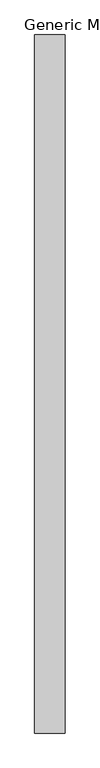
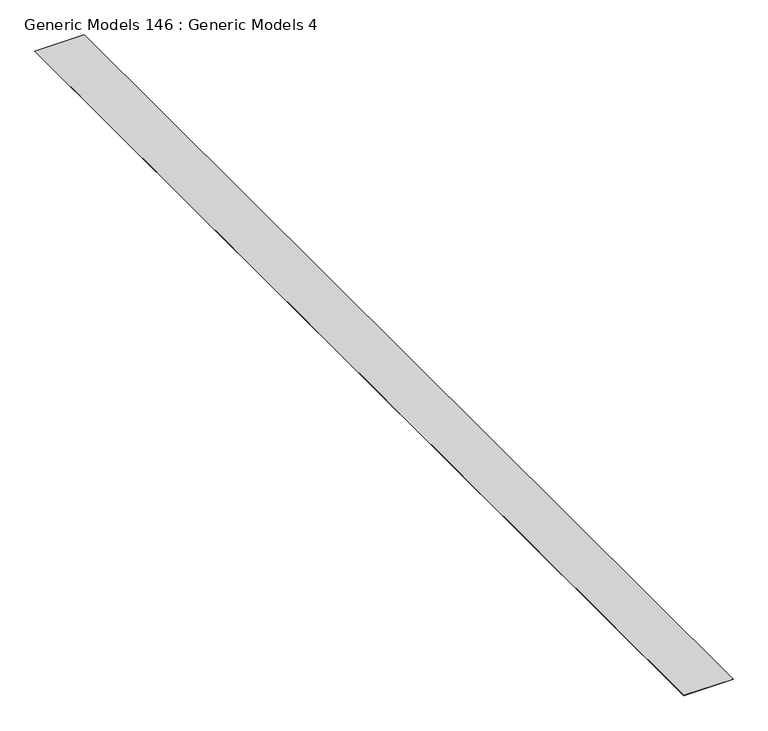
"""IFC4 building model written with IfcOpenShell, lengths in millimetres: proxy geometry, Generic Models 146 : Generic Models 4."""

from ifc_helpers import new_model, si_unit, frame, origin, place, context, project, spatial, polyline, outline, extrude, source, transform, mapped, element, save


def generic_models_146_generic_models_4_f75732ef(model_context):
    return source(origin(), model_context, "Body", "SweptSolid", [
        extrude(outline(polyline([(-5950.1236296, -5493.3230338), (-6498.6122941, -5493.3230338), (-6498.6122941, 7054.2769662), (-5950.1236296, 7054.2769662), (-5950.1236296, -5493.3230338)])), frame((0.0, 0.0, 123259.596), z_axis=(0.0, 0.0, 1.0), x_axis=(1.0, 0.0, 0.0)), (0.0, 0.0, 1.0), 1.5875),
    ])


if __name__ == "__main__":
    model = new_model("IFC4")
    model_context = context("Model", 3, world=origin())
    ifc_project = project(units=[si_unit("LENGTHUNIT", "METRE", prefix="MILLI")], contexts=[model_context])
    site = spatial("IfcSite", under=ifc_project)
    building = spatial("IfcBuilding", under=site)
    placement = place(None, origin())
    generic_models_146_generic_models_4_shape = generic_models_146_generic_models_4_f75732ef(model_context)
    element("IfcBuildingElementProxy", 1, Name="Generic Models 146 : Generic Models 4", ObjectType="Generic Models 146 : Generic Models 4", at=placement, inside=building, context=model_context, shape_type="MappedRepresentation", body=[
        mapped(generic_models_146_generic_models_4_shape, transform((0.0, 0.0, 0.0), x_axis=(1.0, 0.0, 0.0), y_axis=(0.0, 1.0, 0.0), z_axis=(0.0, 0.0, 1.0))),
    ])
    save(model, "model.ifc")

# Revit data of these elements
# Element 1 (IfcBuildingElementProxy, "Generic Models 146 : Generic Models 4")
#   Materials on its faces: "_6 MIL VAPOR BARRIER"
# Materials
#   "_6 MIL VAPOR BARRIER": class "Generic", colour RGB 67 154 161, transparency 0, Cost = 0
